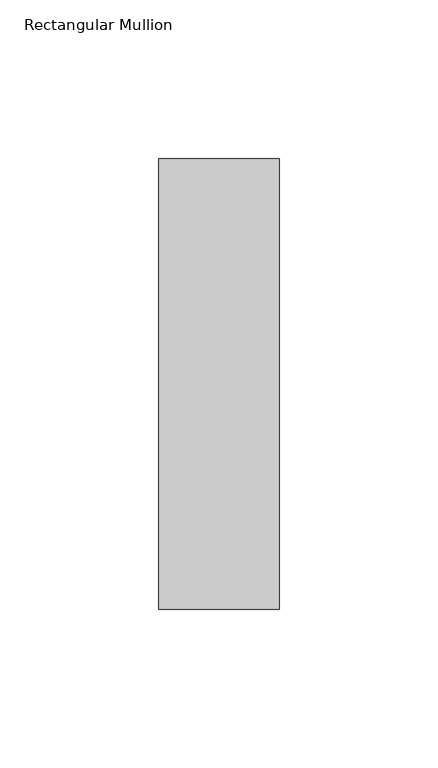
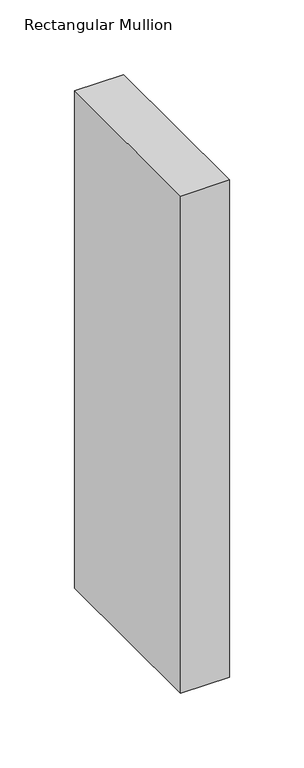
"""IFC4 building model written with IfcOpenShell, lengths in millimetres: member geometry, Rectangular Mullion : NLRS_21_CWM_hsb-regel 38x142_gen_rsf."""

from ifc_helpers import new_model, si_unit, frame, origin, place, context, project, spatial, polyline, outline, extrude, source, transform, mapped, element, save


def rectangular_mullion_fd8aedfe(model_context):
    return source(origin(), model_context, "Body", "SweptSolid", [
        extrude(outline(polyline([(-38.0, -71.0), (-38.0, 71.0), (0.0, 71.0), (0.0, -71.0), (-38.0, -71.0)])), frame((0.0, 0.0, -407.0), z_axis=(0.0, 0.0, 1.0), x_axis=(1.0, 0.0, 0.0)), (0.0, 0.0, 1.0), 407.0),
    ])


if __name__ == "__main__":
    model = new_model("IFC4")
    model_context = context("Model", 3, world=origin())
    ifc_project = project(units=[si_unit("LENGTHUNIT", "METRE", prefix="MILLI")], contexts=[model_context])
    site = spatial("IfcSite", under=ifc_project)
    building = spatial("IfcBuilding", under=site)
    placement = place(None, origin())
    rectangular_mullion_shape = rectangular_mullion_fd8aedfe(model_context)
    element("IfcMember", 1, ObjectType="Rectangular Mullion : NLRS_21_CWM_hsb-regel 38x142_gen_rsf", at=placement, inside=building, context=model_context, shape_type="MappedRepresentation", body=[
        mapped(rectangular_mullion_shape, transform((0.0, 0.0, 0.0), x_axis=(1.0, 0.0, 0.0), y_axis=(0.0, 1.0, 0.0), z_axis=(0.0, 0.0, 1.0))),
    ])
    save(model, "model.ifc")

# Revit data of these elements
# Type "Rectangular Mullion : NLRS_21_CWM_hsb-regel 38x142_gen_rsf"
#   Export Type to IFC As = "IfcWall"
#   Type IfcGUID = "07M7mRoiH1CR8m_RSKIwpF"
#   Assembly Code = "21.10"
#   built-in parameter 1007322 = 0.465879 (stored number, unit not read)
#   built-in parameter 1007321 = 0.062336 (stored number, unit not read)
#   built-in parameter 1007320 = 0.062336 (stored number, unit not read)
# Element 1 (IfcMember, "Rectangular Mullion : NLRS_21_CWM_hsb-regel 38x142_gen_rsf")
#   Materials on its faces: "NLRS_i2_hout naaldhout vuren_gen_rsf"
# Materials
#   "NLRS_i2_hout naaldhout vuren_gen_rsf": class "I - Hout", colour RGB 234 199 147, transparency 0, Keynote = "i2", Manufacturer = "Revit Standards Foundation", URL = "www.revitstandards.org", Description = "hout vuren", Cost = 0
